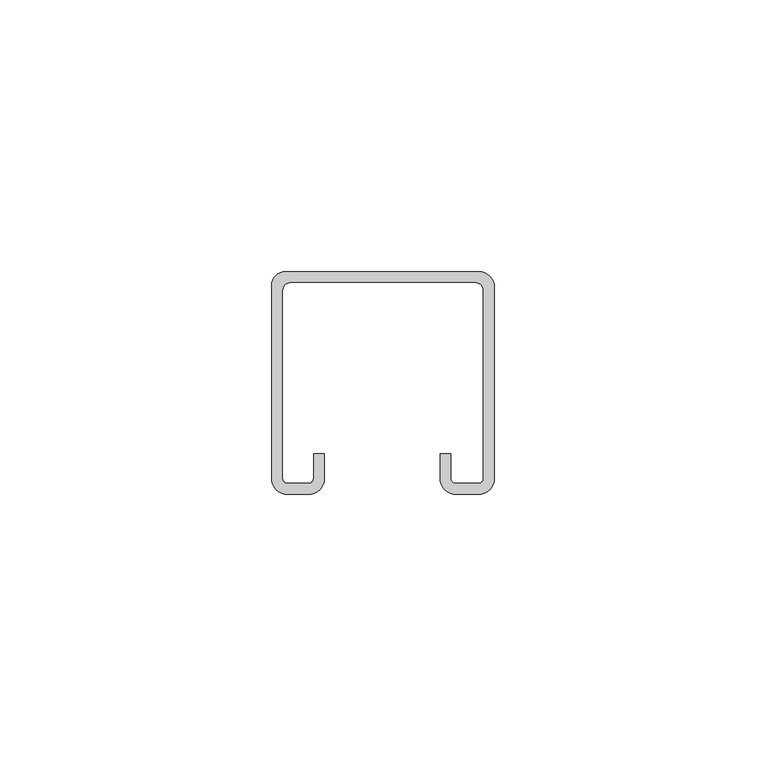
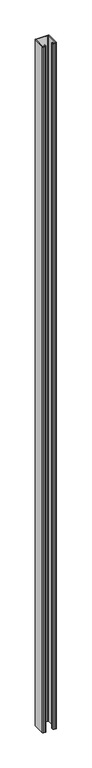
"""IFC4 building model written with IfcOpenShell, lengths in millimetres: proxy geometry, TN_Профиль монтажный : Профиль монтажный 41х41x2,0-3000."""

from ifc_helpers import new_model, si_unit, point, frame_2d, origin, origin_with_axes, place, context, project, spatial, polyline, circle_curve, trimmed, segment, composite_curve, outline, extrude, source, transform, mapped, element, save


def generic_models_78ab1951(model_context):
    return source(origin(), model_context, "Body", "SweptSolid", [
        extrude(outline(composite_curve([segment(polyline([(20.7157599, -2.9315199), (20.7157599, -38.0)]), True, "CONTINUOUS"), segment(trimmed(circle_curve(frame_2d((17.7157599, -38.0)), 3.0), [point((20.7157599, -38.0))], [point((17.7157599, -41.0))], False, "CARTESIAN"), True, "CONTINUOUS"), segment(polyline([(17.7157599, -41.0), (13.7568638, -41.0)]), True, "CONTINUOUS"), segment(trimmed(circle_curve(frame_2d((13.7568638, -37.9588961)), 3.0411039), [point((13.7568638, -41.0))], [point((10.7157599, -37.9588961))], False, "CARTESIAN"), True, "CONTINUOUS"), segment(polyline([(10.7157599, -37.9588961), (10.7157599, -33.5), (12.7157599, -33.5), (12.7157599, -38.0)]), True, "CONTINUOUS"), segment(trimmed(circle_curve(frame_2d((13.7157599, -38.0)), 1.0), [point((12.7157599, -38.0))], [point((13.7157599, -39.0))], True, "CARTESIAN"), True, "CONTINUOUS"), segment(polyline([(13.7157599, -39.0), (17.7157599, -39.0)]), True, "CONTINUOUS"), segment(trimmed(circle_curve(frame_2d((17.7157599, -38.0)), 1.0), [point((17.7157599, -39.0))], [point((18.7157599, -38.0))], True, "CARTESIAN"), True, "CONTINUOUS"), segment(polyline([(18.7157599, -38.0), (18.7157599, -3.5)]), True, "CONTINUOUS"), segment(trimmed(circle_curve(frame_2d((17.2157599, -3.5)), 1.5), [point((18.7157599, -3.5))], [point((17.2157599, -2.0))], True, "CARTESIAN"), True, "CONTINUOUS"), segment(polyline([(17.2157599, -2.0), (-16.7842401, -2.0)]), True, "CONTINUOUS"), segment(trimmed(circle_curve(frame_2d((-16.7842401, -3.5)), 1.5), [point((-16.7842401, -2.0))], [point((-18.2842401, -3.5))], True, "CARTESIAN"), True, "CONTINUOUS"), segment(polyline([(-18.2842401, -3.5), (-18.2842401, -38.0)]), True, "CONTINUOUS"), segment(trimmed(circle_curve(frame_2d((-17.2842401, -38.0)), 1.0), [point((-18.2842401, -38.0))], [point((-17.2842401, -39.0))], True, "CARTESIAN"), True, "CONTINUOUS"), segment(polyline([(-17.2842401, -39.0), (-13.5684801, -39.0)]), True, "CONTINUOUS"), segment(trimmed(circle_curve(frame_2d((-13.5684801, -38.0)), 1.0), [point((-13.5684801, -39.0))], [point((-12.5684801, -38.0))], True, "CARTESIAN"), True, "CONTINUOUS"), segment(polyline([(-12.5684801, -38.0), (-12.5684801, -33.5), (-10.5684801, -33.5), (-10.5684801, -38.0)]), True, "CONTINUOUS"), segment(trimmed(circle_curve(frame_2d((-13.5684801, -38.0)), 3.0), [point((-10.5684801, -38.0))], [point((-13.5684801, -41.0))], False, "CARTESIAN"), True, "CONTINUOUS"), segment(polyline([(-13.5684801, -41.0), (-17.2842401, -41.0)]), True, "CONTINUOUS"), segment(trimmed(circle_curve(frame_2d((-17.2842401, -38.0)), 3.0), [point((-17.2842401, -41.0))], [point((-20.2842401, -38.0))], False, "CARTESIAN"), True, "CONTINUOUS"), segment(polyline([(-20.2842401, -38.0), (-20.2842401, -2.5)]), True, "CONTINUOUS"), segment(trimmed(circle_curve(frame_2d((-17.7842401, -2.5)), 2.5), [point((-20.2842401, -2.5))], [point((-17.7842401, 0.0))], False, "CARTESIAN"), True, "CONTINUOUS"), segment(polyline([(-17.7842401, 0.0), (17.7842401, 0.0)]), True, "CONTINUOUS"), segment(trimmed(circle_curve(frame_2d((17.7842401, -2.9315199)), 2.9315199), [point((17.7842401, 0.0))], [point((20.7157599, -2.9315199))], False, "CARTESIAN"), True, "CONTINUOUS")], self_intersect=False)), origin_with_axes(), (0.0, 0.0, 1.0), 2150.0),
    ])


if __name__ == "__main__":
    model = new_model("IFC4")
    model_context = context("Model", 3, world=origin())
    ifc_project = project(units=[si_unit("LENGTHUNIT", "METRE", prefix="MILLI")], contexts=[model_context])
    site = spatial("IfcSite", under=ifc_project)
    building = spatial("IfcBuilding", under=site)
    placement = place(None, origin())
    generic_models_shape = generic_models_78ab1951(model_context)
    element("IfcBuildingElementProxy", 1, Name="TN_Профиль монтажный : Профиль монтажный 41х41x2,0-3000", ObjectType="TN_Профиль монтажный : Профиль монтажный 41х41x2,0-3000", at=placement, inside=building, context=model_context, shape_type="MappedRepresentation", body=[
        mapped(generic_models_shape, transform((0.0, 0.0, 0.0), x_axis=(1.0, 0.0, 0.0), y_axis=(0.0, 1.0, 0.0), z_axis=(0.0, 0.0, 1.0))),
    ])
    save(model, "model.ifc")

# Revit data of these elements
# Type "TN_Профиль монтажный : Профиль монтажный 41х41x2,0-3000"
#   Description = "Профиль монтажный – траверса С-образной формы предназначен для горизонтального и вертикального монтажа тяжелых инженерных систем, оборудования систем вентиляции и кондиционирования, установок электроснабжения, элементов трубопроводов, также для изготовления стенных консолей пристенного монтажа, рам оснований различного типа под оборудование. Возможно замещение на основе сконструированных модулей серийных опор ГОСТ для раскрепления технологических трубопроводов. Рекомендуется для применения в сухих, влажных помещениях и на открытом воздухе."
#   Manufacturer = "ТехноНИКОЛЬ"
#   Model = "Комплектующие к опорам"
#   URL = "https://nav.tn.ru/knowledge-base/polimernye-membrany/opory-pod-oborudovanie-na-ploskoy-krovle/?sphrase_id=266812"
#   ADSK_Обозначение = "ТехноНИКОЛЬ"
#   ADSK_Наименование краткое = "П41х41x2,0"
#   ADSK_Наименование = "Профиль монтажный 41х41x2,0-3000"
#   ADSK_Масса_Текст = ""
#   ADSK_Марка = "П41х41x2,0"
#   ADSK_Код изделия = "660816"
#   ADSK_Завод-изготовитель = "ТехноНИКОЛЬ"
#   ADSK_Единица измерения = "п.м."
#   ADSK_Группирование = "Комплектующие к опорам"
#   ADSK_URL страницы изделия = "https://nav.tn.ru/knowledge-base/polimernye-membrany/opory-pod-oborudovanie-na-ploskoy-krovle/?sphrase_id=266812"
#   ADSK_URL документации изделия = ""
#   Размер_Длина_Вводимая [instance default] = 1000 mm
#   ADSK_Размер_Длина [instance default] = 1000 mm
#   ADSK_Количество [instance default] = 1
#   Тип профиля = 1
#   Профиль монтажный 41х41x2,0 = yes
#   Профиль монтажный 41x62x2,5 = no
#   Профиль монтажный 41x124x2,5 = no
#   ADSK_Материал = TN_СтальГальванизированная_Серый
#   Default Elevation = 0
# Element 1 (IfcBuildingElementProxy, "TN_Профиль монтажный : Профиль монтажный 41х41x2,0-3000")
#   Размер_Длина_Вводимая = 2150 mm
#   ADSK_Размер_Длина = 2150 mm
#   ADSK_Количество = 2.15
#   Materials on its faces: "TN_СтальГальванизированная_Серый"
# Materials
#   "TN_СтальГальванизированная_Серый": class "Типовые", colour RGB 206 210 213, transparency 0, Cost = 0
